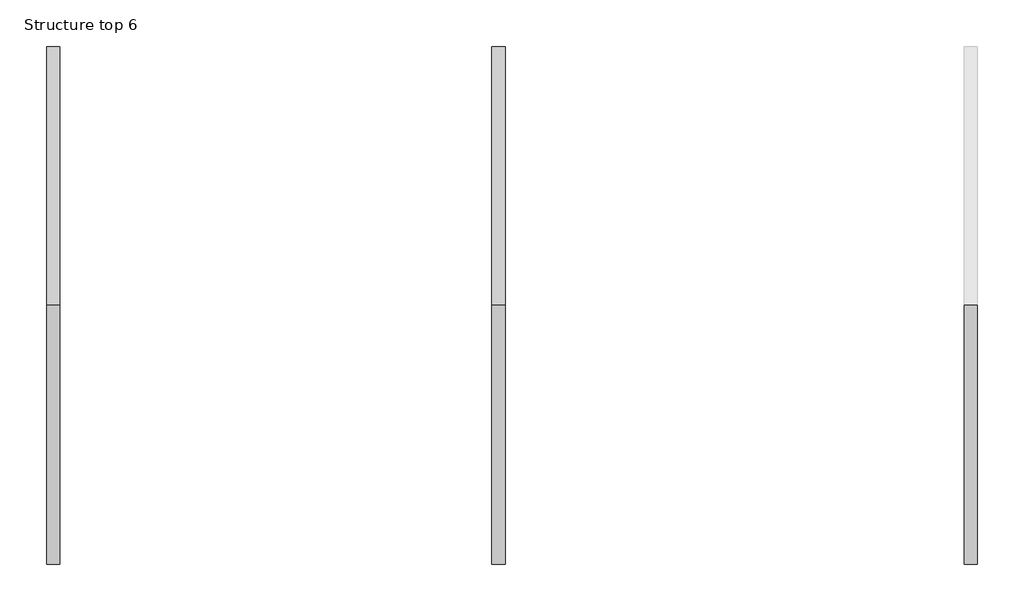
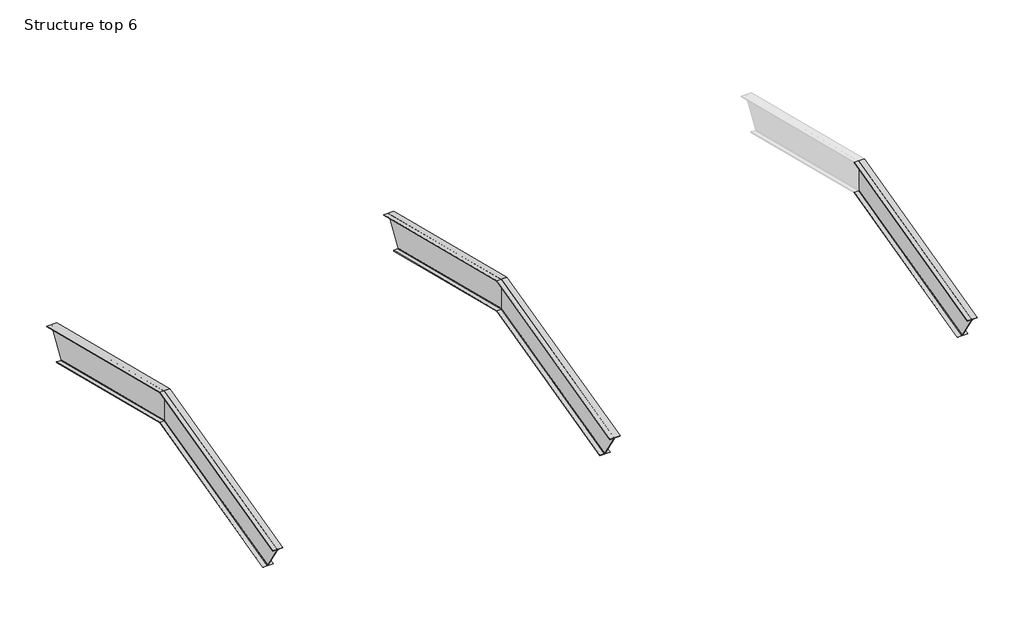
# One storey, part 1 of 2: 5 beams.
"""IFC4 building model written with IfcOpenShell, lengths in millimetres."""

import ifcopenshell
import ifcopenshell.guid

model = None  # the IFC model being written
_history = None  # IfcOwnerHistory: only IFC2X3 demands one
_inside = {}  # id of a spatial element -> (the spatial element, [elements in it])
_under = {}  # id of a project, library or spatial element -> (it, [spatial elements below it])
_declared = {}  # id of a project -> (the project, [libraries it declares])
_typed = {}  # id of a type object -> (the type object, [elements of that type])
_made_of = {}  # id of a material, layer set ... -> (it, [elements and type objects made of it])


def new_model(schema):
    """Start an empty IFC model of exactly this schema.

    Asked for "IFC4X3", IfcOpenShell would pick the latest addendum, in which some entities
    have other attributes; the version numbers below select the first issue.
    IFC2X3 requires an IfcOwnerHistory on every rooted entity: one is made here for all.
    """
    global model, _history
    if schema == "IFC4X3":
        model = ifcopenshell.file(schema_version=(4, 3, 0, 0))
    else:
        model = ifcopenshell.file(schema=schema)
    _inside.clear()
    _under.clear()
    _declared.clear()
    _typed.clear()
    _made_of.clear()
    _history = None
    if model.schema == "IFC2X3":
        org = make("IfcOrganization", Name="unknown")
        user = make(
            "IfcPersonAndOrganization",
            ThePerson=make("IfcPerson", FamilyName="unknown"),
            TheOrganization=org,
        )
        app = make(
            "IfcApplication",
            ApplicationDeveloper=org,
            Version="unknown",
            ApplicationFullName="unknown",
            ApplicationIdentifier="unknown",
        )
        _history = make(
            "IfcOwnerHistory",
            OwningUser=user,
            OwningApplication=app,
            ChangeAction="ADDED",
            CreationDate=0,
        )
    return model


def make(cls, **values):
    """One entity of the class cls with the attributes given. An attribute that is None is left unset."""
    return model.create_entity(
        cls, **{name: value for name, value in values.items() if value is not None}
    )


def rooted(cls, **values):
    """An entity with a GlobalId (a new one), such as an element, a storey or a relation."""
    return make(cls, GlobalId=ifcopenshell.guid.new(), OwnerHistory=_history, **values)


def si_unit(unit_type, name, prefix=None):
    """IfcSIUnit, for example si_unit("LENGTHUNIT", "METRE", prefix="MILLI")."""
    return make("IfcSIUnit", UnitType=unit_type, Prefix=prefix, Name=name)


def assignment(units):
    """IfcUnitAssignment: the units of a project."""
    return None if units is None else make("IfcUnitAssignment", Units=units)


def point(xyz):
    """IfcCartesianPoint."""
    return None if xyz is None else make("IfcCartesianPoint", Coordinates=xyz)


def direction(xyz):
    """IfcDirection."""
    return None if xyz is None else make("IfcDirection", DirectionRatios=xyz)


def frame(location, z_axis=None, x_axis=None):
    """IfcAxis2Placement3D, a coordinate frame: its origin and axes. An axis left out is left unset."""
    return make(
        "IfcAxis2Placement3D",
        Location=point(location),
        Axis=direction(z_axis),
        RefDirection=direction(x_axis),
    )


def origin():
    """The frame at (0, 0, 0) with its axes left unset."""
    return frame((0.0, 0.0, 0.0))


def place(relative_to, where):
    """IfcLocalPlacement: puts the frame where relative to a parent placement (None: the world)."""
    return make(
        "IfcLocalPlacement", PlacementRelTo=relative_to, RelativePlacement=where
    )


def context(
    kind, dimensions, precision=None, world=None, true_north=None, identifier=None
):
    """IfcGeometricRepresentationContext, for example the 3D "Model" context."""
    return make(
        "IfcGeometricRepresentationContext",
        ContextIdentifier=identifier,
        ContextType=kind,
        CoordinateSpaceDimension=dimensions,
        Precision=precision,
        WorldCoordinateSystem=world,
        TrueNorth=true_north,
    )


def project(units=None, contexts=None):
    """IfcProject with its units and contexts."""
    return rooted(
        "IfcProject",
        Name="project",
        RepresentationContexts=contexts,
        UnitsInContext=assignment(units),
    )


def spatial(cls, under=None, at=None, **own):
    """A site, building, storey or space (cls), placed at a placement, below another one or the project."""
    s = rooted(cls, ObjectPlacement=at, **own)
    if under is not None:
        _under.setdefault(under.id(), (under, []))[1].append(s)
    return s


def polyline(points):
    """IfcPolyline through the points."""
    return make("IfcPolyline", Points=[point(p) for p in points])


def ellipse_curve(where, semi_axis1, semi_axis2):
    """IfcEllipse in the frame where."""
    return make(
        "IfcEllipse", Position=where, SemiAxis1=semi_axis1, SemiAxis2=semi_axis2
    )


def shape(context_of_items, identifier, shape_type, items):
    """IfcShapeRepresentation: the items that make up one representation, for example the "Body"."""
    return make(
        "IfcShapeRepresentation",
        ContextOfItems=context_of_items,
        RepresentationIdentifier=identifier,
        RepresentationType=shape_type,
        Items=items,
    )


def made_of(thing, what):
    """Note that an element or type object is made of a material, layer set ...; save() writes the relation."""
    if what is not None:
        _made_of.setdefault(what.id(), (what, []))[1].append(thing)
    return thing


def element(
    cls,
    number,
    at=None,
    inside=None,
    cuts=None,
    type_object=None,
    material=None,
    context=None,
    identifier="Body",
    shape_type=None,
    held_by="IfcProductDefinitionShape",
    body=None,
    shapes=None,
    **own,
):
    """One element of the class cls, such as IfcWall. Its Tag is "e" and its number.

    at: its placement. inside: the storey or other place that contains it. cuts: it is an
    opening in that element (IfcRelVoidsElement). A single representation is given by context,
    identifier, shape_type and body (its items); several are given by shapes. held_by: the class
    of the entity that holds the representations. save() writes the other relations.
    """
    e = rooted(cls, Tag="e%d" % number, ObjectPlacement=at, **own)
    if body is not None:
        shapes = [shape(context, identifier, shape_type, body)]
    if shapes is not None:
        e.Representation = make(held_by, Representations=shapes)
    if inside is not None:
        _inside.setdefault(inside.id(), (inside, []))[1].append(e)
    if cuts is not None:
        rooted(
            "IfcRelVoidsElement", RelatingBuildingElement=cuts, RelatedOpeningElement=e
        )
    if type_object is not None:
        _typed.setdefault(type_object.id(), (type_object, []))[1].append(e)
    return made_of(e, material)


def aggregate(whole, parts):
    """IfcRelAggregates: a whole, such as a stair, and the parts it consists of."""
    return rooted("IfcRelAggregates", RelatingObject=whole, RelatedObjects=parts)


def save(model, path):
    """Write the relations noted so far, then the file.

    IfcRelAggregates (storeys below a building ...), IfcRelContainedInSpatialStructure (elements
    in a storey), IfcRelDefinesByType, IfcRelAssociatesMaterial and IfcRelDeclares: one each for
    every whole, place, type object, material and project.
    """
    for whole, parts in _under.values():
        aggregate(whole, parts)
    for where, things in _inside.values():
        rooted(
            "IfcRelContainedInSpatialStructure",
            RelatedElements=things,
            RelatingStructure=where,
        )
    for kind, things in _typed.values():
        rooted("IfcRelDefinesByType", RelatedObjects=things, RelatingType=kind)
    for what, things in _made_of.values():
        rooted("IfcRelAssociatesMaterial", RelatedObjects=things, RelatingMaterial=what)
    for by, libraries in _declared.values():
        rooted("IfcRelDeclares", RelatingContext=by, RelatedDefinitions=libraries)
    model.write(path)


def plane_surface(at):
    """IfcPlane: the flat surface through the origin of the frame at, square to its z axis."""
    return make("IfcPlane", Position=at)


def revolved_surface(curve, axis_point, axis_direction):
    """IfcSurfaceOfRevolution: the curve turned about the line through axis_point along axis_direction."""
    return make(
        "IfcSurfaceOfRevolution",
        SweptCurve=make("IfcArbitraryOpenProfileDef", ProfileType="CURVE", Curve=curve),
        AxisPosition=make("IfcAxis1Placement", Location=point(axis_point), Axis=direction(axis_direction)),
    )


def advanced_brep(points, edges, surfaces, faces):
    """IfcAdvancedBrep: a solid bounded by faces that lie on surfaces and meet in shared edges.

    An edge is (start, end): straight between two places in points (the first is 0);
    or (start, end, curve); or (start, end, curve, False) where it runs against its curve.
    A face is (place in surfaces, loops), or (place, loops, False) where it looks against
    its surface's normal. A loop lists edges by number (the first is 1), with a minus sign
    where the edge is run from its end to its start. The first loop is the outer one.
    """
    corners = [point(p) for p in points]
    vertices = [make("IfcVertexPoint", VertexGeometry=c) for c in corners]
    made = []
    for start, end, *more in edges:
        made.append(
            make(
                "IfcEdgeCurve",
                EdgeStart=vertices[start],
                EdgeEnd=vertices[end],
                EdgeGeometry=more[0] if more else make("IfcPolyline", Points=[corners[start], corners[end]]),
                SameSense=more[1] if len(more) > 1 else True,
            )
        )
    hull = []
    for where, loops, *sense in faces:
        bounds = []
        for j, loop in enumerate(loops):
            ring = [make("IfcOrientedEdge", EdgeElement=made[abs(k) - 1], Orientation=k > 0) for k in loop]
            bounds.append(
                make(
                    "IfcFaceOuterBound" if j == 0 else "IfcFaceBound",
                    Bound=make("IfcEdgeLoop", EdgeList=ring),
                    Orientation=True,
                )
            )
        hull.append(make("IfcAdvancedFace", Bounds=bounds, FaceSurface=surfaces[where], SameSense=sense[0] if sense else True))
    return make("IfcAdvancedBrep", Outer=make("IfcClosedShell", CfsFaces=hull))


model = new_model("IFC4")

# Units and contexts
model_context = context("Model", 3, world=origin())
ifc_project = project(units=[si_unit("LENGTHUNIT", "METRE", prefix="MILLI")], contexts=[model_context])

# Site, building, storey
site = spatial("IfcSite", under=ifc_project)
building = spatial("IfcBuilding", under=site)
storey = spatial("IfcBuildingStorey", under=building, Name="Structure top 6", Elevation=5867.6650904)

# Beams
placement = place(None, origin())
element("IfcBeam", 1, ObjectType="W Shapes : W 6X18.5", at=placement, inside=storey, context=model_context, shape_type="AdvancedBrep", body=[
    advanced_brep(
    [(12635.1244333, 7113.772024, 5183.7974927), (12700.7834333, 7113.772024, 5183.7974927), (12700.7834333, 9790.156119, 4514.7014689), (12635.1244333, 9790.156119, 4514.7014689), (12627.5044333, 7113.772024, 5191.6520089), (12627.5044333, 9794.417492, 4521.4906419), (12627.5044333, 7113.772024, 5640.4067021), (12627.5044333, 10037.8839324, 4909.378725), (12635.1244333, 7113.772024, 5648.2612183), (12635.1244333, 10042.1453053, 4916.1678979), (12700.7834333, 7113.772024, 5648.2612183), (12700.7834333, 10042.1453053, 4916.1678979), (12700.7834333, 7113.772024, 5658.2102722), (12700.7834333, 10047.5430444, 4924.7675171), (12548.3834333, 7113.772024, 5658.2102722), (12548.3834333, 10047.5430444, 4924.7675171), (12548.3834333, 7113.772024, 5648.2612183), (12548.3834333, 10042.1453053, 4916.1678979), (12614.0424333, 7113.772024, 5648.2612183), (12614.0424333, 10042.1453053, 4916.1678979), (12621.6624333, 7113.772024, 5640.4067021), (12621.6624333, 10037.8839324, 4909.378725), (12621.6624333, 7113.772024, 5191.6520089), (12621.6624333, 9794.417492, 4521.4906419), (12614.0424333, 7113.772024, 5183.7974927), (12614.0424333, 9790.156119, 4514.7014689), (12548.3834333, 7113.772024, 5183.7974927), (12548.3834333, 9790.156119, 4514.7014689), (12548.3834333, 7113.772024, 5173.8484388), (12548.3834333, 9784.75838, 4506.1018498), (12700.7834333, 7113.772024, 5173.8484388), (12700.7834333, 9784.75838, 4506.1018498)],
    [
        (0, 1),
        (1, 2),
        (2, 3),
        (3, 0),
        (4, 0, ellipse_curve(frame((12635.1244333, 7113.772024, 5191.6520089), z_axis=(0.0, -1.0, 0.0), x_axis=(0.0, 0.0, -1.0)), 7.8545162, 7.62)),
        (3, 5, ellipse_curve(frame((12635.1244333, 9794.417492, 4521.4906419), z_axis=(0.0, 0.8469796531886633, -0.5316253070390948), x_axis=(0.0, 0.531625307039094, 0.8469796531886635)), 8.0157451, 7.62)),
        (5, 4),
        (6, 4),
        (5, 7),
        (7, 6),
        (8, 6, ellipse_curve(frame((12635.1244333, 7113.772024, 5640.4067021), z_axis=(0.0, -1.0, 0.0), x_axis=(0.0, 0.0, -1.0)), 7.8545162, 7.62)),
        (7, 9, ellipse_curve(frame((12635.1244333, 10037.8839324, 4909.378725), z_axis=(0.0, 0.8469796531886633, -0.5316253070390948), x_axis=(0.0, 0.531625307039094, 0.8469796531886635)), 8.0157451, 7.62)),
        (9, 8),
        (10, 8),
        (9, 11),
        (11, 10),
        (12, 10),
        (11, 13),
        (13, 12),
        (14, 12),
        (13, 15),
        (15, 14),
        (16, 14),
        (15, 17),
        (17, 16),
        (18, 16),
        (17, 19),
        (19, 18),
        (20, 18, ellipse_curve(frame((12614.0424333, 7113.772024, 5640.4067021), z_axis=(0.0, -1.0, 0.0), x_axis=(0.0, 0.0, -1.0)), 7.8545162, 7.62)),
        (19, 21, ellipse_curve(frame((12614.0424333, 10037.8839324, 4909.378725), z_axis=(0.0, 0.8469796531886633, -0.5316253070390948), x_axis=(0.0, 0.531625307039094, 0.8469796531886635)), 8.0157451, 7.62)),
        (21, 20),
        (22, 20),
        (21, 23),
        (23, 22),
        (24, 22, ellipse_curve(frame((12614.0424333, 7113.772024, 5191.6520089), z_axis=(0.0, -1.0, 0.0), x_axis=(0.0, 0.0, -1.0)), 7.8545162, 7.62)),
        (23, 25, ellipse_curve(frame((12614.0424333, 9794.417492, 4521.4906419), z_axis=(0.0, 0.8469796531886633, -0.5316253070390948), x_axis=(0.0, 0.531625307039094, 0.8469796531886635)), 8.0157451, 7.62)),
        (25, 24),
        (26, 24),
        (25, 27),
        (27, 26),
        (28, 26),
        (27, 29),
        (29, 28),
        (30, 28),
        (29, 31),
        (31, 30),
        (1, 30),
        (31, 2),
    ],
    [
        plane_surface(frame((12700.7834333, 7002.1447176, 5211.7043193), z_axis=(0.0, 0.24253562503633289, 0.9701425001453319), x_axis=(0.0, 0.9701425001453319, -0.24253562503633289))),
        revolved_surface(polyline([(12627.504433299999, 9796.830743469387, 4520.887328982653), (12627.504433299999, 7111.923902529412, 5192.114039217647)]), (12635.1244333, 7003.992839, 5219.0968051), (0.0, 0.9701425001453319, -0.24253562503633289)),
        plane_surface(frame((12627.5044333, 7003.992839, 5219.0968051), z_axis=(1.0, 0.0, 0.0), x_axis=(0.0, 0.9701425001453319, -0.24253562503633289))),
        revolved_surface(polyline([(12627.504433299999, 10040.297183869387, 4908.775412082653), (12627.504433299999, 7111.923902529412, 5640.868732417647)]), (12635.1244333, 7109.5821786, 5641.4541634), (0.0, 0.9701425001453319, -0.24253562503633289)),
        plane_surface(frame((12635.1244333, 7111.4303001, 5648.8466493), z_axis=(0.0, -0.24253562503633289, -0.9701425001453319), x_axis=(0.0, 0.9701425001453319, -0.24253562503633289))),
        plane_surface(frame((12700.7834333, 7111.4303001, 5648.8466493), z_axis=(1.0, 0.0, 0.0), x_axis=(0.0, 0.9701425001453319, -0.24253562503633289))),
        plane_surface(frame((12700.7834333, 7113.7712539, 5658.2104647), z_axis=(0.0, 0.24253562503633289, 0.9701425001453319), x_axis=(0.0, 0.9701425001453319, -0.24253562503633289))),
        plane_surface(frame((12548.3834333, 7113.7712539, 5658.2104647), z_axis=(-1.0, 0.0, 0.0), x_axis=(0.0, 0.9701425001453319, -0.24253562503633289))),
        plane_surface(frame((12548.3834333, 7111.4303001, 5648.8466493), z_axis=(0.0, -0.24253562503633289, -0.9701425001453319), x_axis=(0.0, 0.9701425001453319, -0.24253562503633289))),
        revolved_surface(polyline([(12606.422433299998, 10040.297183869387, 4908.775412082653), (12606.422433299998, 7111.923902529412, 5640.868732417647)]), (12614.0424333, 7109.5821786, 5641.4541634), (0.0, 0.9701425001453319, -0.24253562503633289)),
        plane_surface(frame((12621.6624333, 7109.5821786, 5641.4541634), z_axis=(-1.0, 0.0, 0.0), x_axis=(0.0, 0.9701425001453319, -0.24253562503633289))),
        revolved_surface(polyline([(12606.422433299998, 9796.830743469387, 4520.887328982653), (12606.422433299998, 7111.923902529412, 5192.114039217647)]), (12614.0424333, 7003.992839, 5219.0968051), (0.0, 0.9701425001453319, -0.24253562503633289)),
        plane_surface(frame((12614.0424333, 7002.1447176, 5211.7043193), z_axis=(0.0, 0.24253562503633289, 0.9701425001453319), x_axis=(0.0, 0.9701425001453319, -0.24253562503633289))),
        plane_surface(frame((12548.3834333, 7002.1447176, 5211.7043193), z_axis=(-1.0, 0.0, 0.0), x_axis=(0.0, 0.9701425001453319, -0.24253562503633289))),
        plane_surface(frame((12548.3834333, 6999.8037637, 5202.3405039), z_axis=(0.0, -0.24253562503633289, -0.9701425001453319), x_axis=(0.0, 0.9701425001453319, -0.24253562503633289))),
        plane_surface(frame((12700.7834333, 6999.8037637, 5202.3405039), z_axis=(1.0, 0.0, 0.0), x_axis=(0.0, 0.9701425001453319, -0.24253562503633289))),
        plane_surface(frame((12624.5870052, 7113.772024, 5658.2135449), z_axis=(0.0, -1.0, 0.0), x_axis=(0.0, 0.0, 1.0))),
        plane_surface(frame((12624.5870052, 10047.54482, 4924.7703459), z_axis=(0.0, 0.8469796531886633, -0.5316253070390948), x_axis=(1.0, 0.0, 0.0))),
    ],
    [
        (0, [[1, 2, 3, 4]]),
        (1, [[5, -4, 6, 7]]),
        (2, [[8, -7, 9, 10]]),
        (3, [[11, -10, 12, 13]]),
        (4, [[14, -13, 15, 16]]),
        (5, [[17, -16, 18, 19]]),
        (6, [[20, -19, 21, 22]]),
        (7, [[23, -22, 24, 25]]),
        (8, [[26, -25, 27, 28]]),
        (9, [[29, -28, 30, 31]]),
        (10, [[32, -31, 33, 34]]),
        (11, [[35, -34, 36, 37]]),
        (12, [[38, -37, 39, 40]]),
        (13, [[41, -40, 42, 43]]),
        (14, [[44, -43, 45, 46]]),
        (15, [[47, -46, 48, -2]]),
        (16, [[-1, -5, -8, -11, -14, -17, -20, -23, -26, -29, -32, -35, -38, -41, -44, -47]]),
        (17, [[-48, -45, -42, -39, -36, -33, -30, -27, -24, -21, -18, -15, -12, -9, -6, -3]]),
    ],
),
])
element("IfcBeam", 2, ObjectType="W Shapes : W 6X18.5", at=placement, inside=storey, context=model_context, shape_type="AdvancedBrep", body=[
    advanced_brep(
    [(12635.1244333, 4437.3879289, 4514.7014689), (12700.7834333, 4437.3879289, 4514.7014689), (12700.7834333, 7113.772024, 5183.7974927), (12635.1244333, 7113.772024, 5183.7974927), (12627.5044333, 4433.1265559, 4521.4906419), (12627.5044333, 7113.772024, 5191.6520089), (12627.5044333, 4189.6601155, 4909.378725), (12627.5044333, 7113.772024, 5640.4067021), (12635.1244333, 4185.3987426, 4916.1678979), (12635.1244333, 7113.772024, 5648.2612183), (12700.7834333, 4185.3987426, 4916.1678979), (12700.7834333, 7113.772024, 5648.2612183), (12700.7834333, 4180.0010035, 4924.7675171), (12700.7834333, 7113.772024, 5658.2102722), (12548.3834333, 4180.0010035, 4924.7675171), (12548.3834333, 7113.772024, 5658.2102722), (12548.3834333, 4185.3987426, 4916.1678979), (12548.3834333, 7113.772024, 5648.2612183), (12614.0424333, 4185.3987426, 4916.1678979), (12614.0424333, 7113.772024, 5648.2612183), (12621.6624333, 4189.6601155, 4909.378725), (12621.6624333, 7113.772024, 5640.4067021), (12621.6624333, 4433.1265559, 4521.4906419), (12621.6624333, 7113.772024, 5191.6520089), (12614.0424333, 4437.3879289, 4514.7014689), (12614.0424333, 7113.772024, 5183.7974927), (12548.3834333, 4437.3879289, 4514.7014689), (12548.3834333, 7113.772024, 5183.7974927), (12548.3834333, 4442.7856679, 4506.1018498), (12548.3834333, 7113.772024, 5173.8484388), (12700.7834333, 4442.7856679, 4506.1018498), (12700.7834333, 7113.772024, 5173.8484388)],
    [
        (0, 1),
        (1, 2),
        (2, 3),
        (3, 0),
        (4, 0, ellipse_curve(frame((12635.1244333, 4433.1265559, 4521.4906419), z_axis=(0.0, -0.8469796531886659, -0.5316253070390907), x_axis=(0.0, 0.5316253070390901, -0.8469796531886661)), 8.0157451, 7.62)),
        (3, 5, ellipse_curve(frame((12635.1244333, 7113.772024, 5191.6520089), z_axis=(0.0, 1.0, 0.0), x_axis=(0.0, 0.0, 0.9999999999999999)), 7.8545162, 7.62)),
        (5, 4),
        (6, 4),
        (5, 7),
        (7, 6),
        (8, 6, ellipse_curve(frame((12635.1244333, 4189.6601155, 4909.378725), z_axis=(0.0, -0.8469796531886659, -0.5316253070390907), x_axis=(0.0, 0.5316253070390901, -0.8469796531886661)), 8.0157451, 7.62)),
        (7, 9, ellipse_curve(frame((12635.1244333, 7113.772024, 5640.4067021), z_axis=(0.0, 1.0, 0.0), x_axis=(0.0, 0.0, 0.9999999999999999)), 7.8545162, 7.62)),
        (9, 8),
        (10, 8),
        (9, 11),
        (11, 10),
        (12, 10),
        (11, 13),
        (13, 12),
        (14, 12),
        (13, 15),
        (15, 14),
        (16, 14),
        (15, 17),
        (17, 16),
        (18, 16),
        (17, 19),
        (19, 18),
        (20, 18, ellipse_curve(frame((12614.0424333, 4189.6601155, 4909.378725), z_axis=(0.0, -0.8469796531886659, -0.5316253070390907), x_axis=(0.0, 0.5316253070390901, -0.8469796531886661)), 8.0157451, 7.62)),
        (19, 21, ellipse_curve(frame((12614.0424333, 7113.772024, 5640.4067021), z_axis=(0.0, 1.0, 0.0), x_axis=(0.0, 0.0, 0.9999999999999999)), 7.8545162, 7.62)),
        (21, 20),
        (22, 20),
        (21, 23),
        (23, 22),
        (24, 22, ellipse_curve(frame((12614.0424333, 4433.1265559, 4521.4906419), z_axis=(0.0, -0.8469796531886659, -0.5316253070390907), x_axis=(0.0, 0.5316253070390901, -0.8469796531886661)), 8.0157451, 7.62)),
        (23, 25, ellipse_curve(frame((12614.0424333, 7113.772024, 5191.6520089), z_axis=(0.0, 1.0, 0.0), x_axis=(0.0, 0.0, 0.9999999999999999)), 7.8545162, 7.62)),
        (25, 24),
        (26, 24),
        (25, 27),
        (27, 26),
        (28, 26),
        (27, 29),
        (29, 28),
        (30, 28),
        (29, 31),
        (31, 30),
        (1, 30),
        (31, 2),
    ],
    [
        plane_surface(frame((12700.7834333, 4291.6265344, 4478.2611203), z_axis=(0.0, -0.2425356250363261, 0.9701425001453337), x_axis=(0.0, 0.9701425001453337, 0.2425356250363261))),
        revolved_surface(polyline([(12627.504433299999, 7115.620145464711, 5192.114039241156), (12627.504433299999, 4430.713304430615, 4520.887328982652)]), (12635.1244333, 4289.7784129, 4485.6536061), (0.0, 0.9701425001453337, 0.2425356250363261)),
        plane_surface(frame((12627.5044333, 4289.7784129, 4485.6536061), z_axis=(1.0, 0.0, 0.0), x_axis=(0.0, 0.9701425001453337, 0.2425356250363261))),
        revolved_surface(polyline([(12627.504433299999, 7115.620145464711, 5640.868732441156), (12627.504433299999, 4187.246864030613, 4908.775412082654)]), (12635.1244333, 4184.1890733, 4908.0109644), (0.0, 0.9701425001453337, 0.2425356250363261)),
        plane_surface(frame((12635.1244333, 4182.3409519, 4915.4034503), z_axis=(0.0, 0.2425356250363261, -0.9701425001453337), x_axis=(0.0, 0.9701425001453337, 0.2425356250363261))),
        plane_surface(frame((12700.7834333, 4182.3409519, 4915.4034503), z_axis=(1.0, 0.0, 0.0), x_axis=(0.0, 0.9701425001453337, 0.2425356250363261))),
        plane_surface(frame((12700.7834333, 4179.999998, 4924.7672657), z_axis=(0.0, -0.2425356250363261, 0.9701425001453337), x_axis=(0.0, 0.9701425001453337, 0.2425356250363261))),
        plane_surface(frame((12548.3834333, 4179.999998, 4924.7672657), z_axis=(-1.0, 0.0, 0.0), x_axis=(0.0, 0.9701425001453337, 0.2425356250363261))),
        plane_surface(frame((12548.3834333, 4182.3409519, 4915.4034503), z_axis=(0.0, 0.2425356250363261, -0.9701425001453337), x_axis=(0.0, 0.9701425001453337, 0.2425356250363261))),
        revolved_surface(polyline([(12606.422433299998, 7115.620145464711, 5640.868732441156), (12606.422433299998, 4187.246864030613, 4908.775412082654)]), (12614.0424333, 4184.1890733, 4908.0109644), (0.0, 0.9701425001453337, 0.2425356250363261)),
        plane_surface(frame((12621.6624333, 4184.1890733, 4908.0109644), z_axis=(-1.0, 0.0, 0.0), x_axis=(0.0, 0.9701425001453337, 0.2425356250363261))),
        revolved_surface(polyline([(12606.422433299998, 7115.620145464711, 5192.114039241156), (12606.422433299998, 4430.713304430615, 4520.887328982652)]), (12614.0424333, 4289.7784129, 4485.6536061), (0.0, 0.9701425001453337, 0.2425356250363261)),
        plane_surface(frame((12614.0424333, 4291.6265344, 4478.2611203), z_axis=(0.0, -0.2425356250363261, 0.9701425001453337), x_axis=(0.0, 0.9701425001453337, 0.2425356250363261))),
        plane_surface(frame((12548.3834333, 4291.6265344, 4478.2611203), z_axis=(-1.0, 0.0, 0.0), x_axis=(0.0, 0.9701425001453337, 0.2425356250363261))),
        plane_surface(frame((12548.3834333, 4293.9674882, 4468.8973049), z_axis=(0.0, 0.2425356250363261, -0.9701425001453337), x_axis=(0.0, 0.9701425001453337, 0.2425356250363261))),
        plane_surface(frame((12700.7834333, 4293.9674882, 4468.8973049), z_axis=(1.0, 0.0, 0.0), x_axis=(0.0, 0.9701425001453337, 0.2425356250363261))),
        plane_surface(frame((12624.5870052, 7113.772024, 5658.2135449), z_axis=(0.0, 1.0, 0.0), x_axis=(0.0, 0.0, -1.0))),
        plane_surface(frame((12624.5870052, 4179.999228, 4924.7703459), z_axis=(0.0, -0.8469796531886659, -0.5316253070390907), x_axis=(1.0, 0.0, 0.0))),
    ],
    [
        (0, [[1, 2, 3, 4]]),
        (1, [[5, -4, 6, 7]]),
        (2, [[8, -7, 9, 10]]),
        (3, [[11, -10, 12, 13]]),
        (4, [[14, -13, 15, 16]]),
        (5, [[17, -16, 18, 19]]),
        (6, [[20, -19, 21, 22]]),
        (7, [[23, -22, 24, 25]]),
        (8, [[26, -25, 27, 28]]),
        (9, [[29, -28, 30, 31]]),
        (10, [[32, -31, 33, 34]]),
        (11, [[35, -34, 36, 37]]),
        (12, [[38, -37, 39, 40]]),
        (13, [[41, -40, 42, 43]]),
        (14, [[44, -43, 45, 46]]),
        (15, [[47, -46, 48, -2]]),
        (16, [[-48, -45, -42, -39, -36, -33, -30, -27, -24, -21, -18, -15, -12, -9, -6, -3]]),
        (17, [[-1, -5, -8, -11, -14, -17, -20, -23, -26, -29, -32, -35, -38, -41, -44, -47]]),
    ],
),
])
element("IfcBeam", 3, ObjectType="W Shapes : W 6X18.5", at=placement, inside=storey, context=model_context, shape_type="AdvancedBrep", body=[
    advanced_brep(
    [(7586.8744333, 7113.772024, 5183.7974927), (7652.5334333, 7113.772024, 5183.7974927), (7652.5334333, 9790.156119, 4514.7014689), (7586.8744333, 9790.156119, 4514.7014689), (7579.2544333, 7113.772024, 5191.6520089), (7579.2544333, 9794.417492, 4521.4906419), (7579.2544333, 7113.772024, 5640.4067021), (7579.2544333, 10037.8839324, 4909.378725), (7586.8744333, 7113.772024, 5648.2612183), (7586.8744333, 10042.1453053, 4916.1678979), (7652.5334333, 7113.772024, 5648.2612183), (7652.5334333, 10042.1453053, 4916.1678979), (7652.5334333, 7113.772024, 5658.2102722), (7652.5334333, 10047.5430444, 4924.7675171), (7500.1334333, 7113.772024, 5658.2102722), (7500.1334333, 10047.5430444, 4924.7675171), (7500.1334333, 7113.772024, 5648.2612183), (7500.1334333, 10042.1453053, 4916.1678979), (7565.7924333, 7113.772024, 5648.2612183), (7565.7924333, 10042.1453053, 4916.1678979), (7573.4124333, 7113.772024, 5640.4067021), (7573.4124333, 10037.8839324, 4909.378725), (7573.4124333, 7113.772024, 5191.6520089), (7573.4124333, 9794.417492, 4521.4906419), (7565.7924333, 7113.772024, 5183.7974927), (7565.7924333, 9790.156119, 4514.7014689), (7500.1334333, 7113.772024, 5183.7974927), (7500.1334333, 9790.156119, 4514.7014689), (7500.1334333, 7113.772024, 5173.8484388), (7500.1334333, 9784.75838, 4506.1018498), (7652.5334333, 7113.772024, 5173.8484388), (7652.5334333, 9784.75838, 4506.1018498)],
    [
        (0, 1),
        (1, 2),
        (2, 3),
        (3, 0),
        (4, 0, ellipse_curve(frame((7586.8744333, 7113.772024, 5191.6520089), z_axis=(0.0, -1.0, 0.0), x_axis=(0.0, 0.0, -1.0)), 7.8545162, 7.62)),
        (3, 5, ellipse_curve(frame((7586.8744333, 9794.417492, 4521.4906419), z_axis=(0.0, 0.8469796531886629, -0.5316253070390953), x_axis=(0.0, 0.5316253070390956, 0.8469796531886628)), 8.0157451, 7.62)),
        (5, 4),
        (6, 4),
        (5, 7),
        (7, 6),
        (8, 6, ellipse_curve(frame((7586.8744333, 7113.772024, 5640.4067021), z_axis=(0.0, -1.0, 0.0), x_axis=(0.0, 0.0, -1.0)), 7.8545162, 7.62)),
        (7, 9, ellipse_curve(frame((7586.8744333, 10037.8839324, 4909.378725), z_axis=(0.0, 0.8469796531886629, -0.5316253070390953), x_axis=(0.0, 0.5316253070390956, 0.8469796531886628)), 8.0157451, 7.62)),
        (9, 8),
        (10, 8),
        (9, 11),
        (11, 10),
        (12, 10),
        (11, 13),
        (13, 12),
        (14, 12),
        (13, 15),
        (15, 14),
        (16, 14),
        (15, 17),
        (17, 16),
        (18, 16),
        (17, 19),
        (19, 18),
        (20, 18, ellipse_curve(frame((7565.7924333, 7113.772024, 5640.4067021), z_axis=(0.0, -1.0, 0.0), x_axis=(0.0, 0.0, -1.0)), 7.8545162, 7.62)),
        (19, 21, ellipse_curve(frame((7565.7924333, 10037.8839324, 4909.378725), z_axis=(0.0, 0.8469796531886629, -0.5316253070390953), x_axis=(0.0, 0.5316253070390956, 0.8469796531886628)), 8.0157451, 7.62)),
        (21, 20),
        (22, 20),
        (21, 23),
        (23, 22),
        (24, 22, ellipse_curve(frame((7565.7924333, 7113.772024, 5191.6520089), z_axis=(0.0, -1.0, 0.0), x_axis=(0.0, 0.0, -1.0)), 7.8545162, 7.62)),
        (23, 25, ellipse_curve(frame((7565.7924333, 9794.417492, 4521.4906419), z_axis=(0.0, 0.8469796531886629, -0.5316253070390953), x_axis=(0.0, 0.5316253070390956, 0.8469796531886628)), 8.0157451, 7.62)),
        (25, 24),
        (26, 24),
        (25, 27),
        (27, 26),
        (28, 26),
        (27, 29),
        (29, 28),
        (30, 28),
        (29, 31),
        (31, 30),
        (1, 30),
        (31, 2),
    ],
    [
        plane_surface(frame((7619.7039333, 7002.1447176, 5211.7043193), z_axis=(0.0, 0.24253562503633289, 0.9701425001453319), x_axis=(-1.0, 0.0, 0.0))),
        revolved_surface(polyline([(7579.2544333000005, 9796.830743469387, 4520.887328982653), (7579.2544333000005, 7111.923902529412, 5192.114039217647)]), (7586.8744333, 7003.992839, 5219.0968051), (0.0, 0.9701425001453319, -0.24253562503633289)),
        plane_surface(frame((7579.2544333, 7056.7875088, 5430.2754843), z_axis=(1.0, 0.0, 0.0), x_axis=(0.0, 0.24253562503633308, 0.9701425001453319))),
        revolved_surface(polyline([(7586.8744333, 10042.145305332164, 4916.16789793376), (7586.8744333, 7113.772023992189, 5648.261218268754)]), (7586.8744333, 7109.5821786, 5641.4541634), (0.0, 0.9701425001453319, -0.24253562503633289)),
        plane_surface(frame((7619.7039333, 7111.4303001, 5648.8466493), z_axis=(0.0, -0.24253562503633289, -0.9701425001453319), x_axis=(1.0, 0.0, 0.0))),
        plane_surface(frame((7652.5334333, 7112.600777, 5653.528557), z_axis=(1.0, 0.0, 0.0), x_axis=(0.0, 0.24253562503633308, 0.9701425001453319))),
        plane_surface(frame((7576.3334333, 7113.7712539, 5658.2104647), z_axis=(0.0, 0.24253562503633289, 0.9701425001453319), x_axis=(-1.0, 0.0, 0.0))),
        plane_surface(frame((7500.1334333, 7112.600777, 5653.528557), z_axis=(-1.0, 0.0, 0.0), x_axis=(0.0, -0.24253562503633308, -0.9701425001453319))),
        plane_surface(frame((7532.9629333, 7111.4303001, 5648.8466493), z_axis=(0.0, -0.24253562503633289, -0.9701425001453319), x_axis=(1.0, 0.0, 0.0))),
        revolved_surface(polyline([(7573.4124333, 10040.297183869387, 4908.775412082653), (7573.4124333, 7111.923902529412, 5640.868732417647)]), (7565.7924333, 7109.5821786, 5641.4541634), (0.0, 0.9701425001453319, -0.24253562503633289)),
        plane_surface(frame((7573.4124333, 7056.7875088, 5430.2754843), z_axis=(-1.0, 0.0, 0.0), x_axis=(0.0, -0.24253562503633308, -0.9701425001453319))),
        revolved_surface(polyline([(7565.7924333, 9794.98262200661, 4513.494843131546), (7565.7924333, 7110.075781066635, 5184.721553366539)]), (7565.7924333, 7003.992839, 5219.0968051), (0.0, 0.9701425001453319, -0.24253562503633289)),
        plane_surface(frame((7532.9629333, 7002.1447176, 5211.7043193), z_axis=(0.0, 0.24253562503633289, 0.9701425001453319), x_axis=(-1.0, 0.0, 0.0))),
        plane_surface(frame((7500.1334333, 7000.9742406, 5207.0224116), z_axis=(-1.0, 0.0, 0.0), x_axis=(0.0, -0.24253562503633308, -0.9701425001453319))),
        plane_surface(frame((7576.3334333, 6999.8037637, 5202.3405039), z_axis=(0.0, -0.24253562503633289, -0.9701425001453319), x_axis=(1.0, 0.0, 0.0))),
        plane_surface(frame((7652.5334333, 7000.9742406, 5207.0224116), z_axis=(1.0, 0.0, 0.0), x_axis=(0.0, 0.24253562503633308, 0.9701425001453319))),
        plane_surface(frame((7576.3370052, 7113.772024, 5658.2135449), z_axis=(0.0, -1.0, 0.0), x_axis=(0.0, 0.0, 1.0))),
        plane_surface(frame((7576.3370052, 10047.54482, 4924.7703459), z_axis=(0.0, 0.8469796531886629, -0.5316253070390953), x_axis=(1.0, 0.0, 0.0))),
    ],
    [
        (0, [[1, 2, 3, 4]]),
        (1, [[5, -4, 6, 7]]),
        (2, [[8, -7, 9, 10]]),
        (3, [[11, -10, 12, 13]]),
        (4, [[14, -13, 15, 16]]),
        (5, [[17, -16, 18, 19]]),
        (6, [[20, -19, 21, 22]]),
        (7, [[23, -22, 24, 25]]),
        (8, [[26, -25, 27, 28]]),
        (9, [[29, -28, 30, 31]]),
        (10, [[32, -31, 33, 34]]),
        (11, [[35, -34, 36, 37]]),
        (12, [[38, -37, 39, 40]]),
        (13, [[41, -40, 42, 43]]),
        (14, [[44, -43, 45, 46]]),
        (15, [[47, -46, 48, -2]]),
        (16, [[-1, -5, -8, -11, -14, -17, -20, -23, -26, -29, -32, -35, -38, -41, -44, -47]]),
        (17, [[-48, -45, -42, -39, -36, -33, -30, -27, -24, -21, -18, -15, -12, -9, -6, -3]]),
    ],
),
])
element("IfcBeam", 4, ObjectType="W Shapes : W 6X18.5", at=placement, inside=storey, context=model_context, shape_type="AdvancedBrep", body=[
    advanced_brep(
    [(7586.8744333, 4437.3879289, 4514.7014689), (7652.5334333, 4437.3879289, 4514.7014689), (7652.5334333, 7113.772024, 5183.7974927), (7586.8744333, 7113.772024, 5183.7974927), (7579.2544333, 4433.1265559, 4521.4906419), (7579.2544333, 7113.772024, 5191.6520089), (7579.2544333, 4189.6601155, 4909.378725), (7579.2544333, 7113.772024, 5640.4067021), (7586.8744333, 4185.3987426, 4916.1678979), (7586.8744333, 7113.772024, 5648.2612183), (7652.5334333, 4185.3987426, 4916.1678979), (7652.5334333, 7113.772024, 5648.2612183), (7652.5334333, 4180.0010035, 4924.7675171), (7652.5334333, 7113.772024, 5658.2102722), (7500.1334333, 4180.0010035, 4924.7675171), (7500.1334333, 7113.772024, 5658.2102722), (7500.1334333, 4185.3987426, 4916.1678979), (7500.1334333, 7113.772024, 5648.2612183), (7565.7924333, 4185.3987426, 4916.1678979), (7565.7924333, 7113.772024, 5648.2612183), (7573.4124333, 4189.6601155, 4909.378725), (7573.4124333, 7113.772024, 5640.4067021), (7573.4124333, 4433.1265559, 4521.4906419), (7573.4124333, 7113.772024, 5191.6520089), (7565.7924333, 4437.3879289, 4514.7014689), (7565.7924333, 7113.772024, 5183.7974927), (7500.1334333, 4437.3879289, 4514.7014689), (7500.1334333, 7113.772024, 5183.7974927), (7500.1334333, 4442.7856679, 4506.1018498), (7500.1334333, 7113.772024, 5173.8484388), (7652.5334333, 4442.7856679, 4506.1018498), (7652.5334333, 7113.772024, 5173.8484388)],
    [
        (0, 1),
        (1, 2),
        (2, 3),
        (3, 0),
        (4, 0, ellipse_curve(frame((7586.8744333, 4433.1265559, 4521.4906419), z_axis=(0.0, -0.8469796531886659, -0.5316253070390907), x_axis=(0.0, 0.5316253070390901, -0.8469796531886661)), 8.0157451, 7.62)),
        (3, 5, ellipse_curve(frame((7586.8744333, 7113.772024, 5191.6520089), z_axis=(0.0, 1.0, 0.0), x_axis=(0.0, 0.0, 0.9999999999999999)), 7.8545162, 7.62)),
        (5, 4),
        (6, 4),
        (5, 7),
        (7, 6),
        (8, 6, ellipse_curve(frame((7586.8744333, 4189.6601155, 4909.378725), z_axis=(0.0, -0.8469796531886659, -0.5316253070390907), x_axis=(0.0, 0.5316253070390901, -0.8469796531886661)), 8.0157451, 7.62)),
        (7, 9, ellipse_curve(frame((7586.8744333, 7113.772024, 5640.4067021), z_axis=(0.0, 1.0, 0.0), x_axis=(0.0, 0.0, 0.9999999999999999)), 7.8545162, 7.62)),
        (9, 8),
        (10, 8),
        (9, 11),
        (11, 10),
        (12, 10),
        (11, 13),
        (13, 12),
        (14, 12),
        (13, 15),
        (15, 14),
        (16, 14),
        (15, 17),
        (17, 16),
        (18, 16),
        (17, 19),
        (19, 18),
        (20, 18, ellipse_curve(frame((7565.7924333, 4189.6601155, 4909.378725), z_axis=(0.0, -0.8469796531886659, -0.5316253070390907), x_axis=(0.0, 0.5316253070390901, -0.8469796531886661)), 8.0157451, 7.62)),
        (19, 21, ellipse_curve(frame((7565.7924333, 7113.772024, 5640.4067021), z_axis=(0.0, 1.0, 0.0), x_axis=(0.0, 0.0, 0.9999999999999999)), 7.8545162, 7.62)),
        (21, 20),
        (22, 20),
        (21, 23),
        (23, 22),
        (24, 22, ellipse_curve(frame((7565.7924333, 4433.1265559, 4521.4906419), z_axis=(0.0, -0.8469796531886659, -0.5316253070390907), x_axis=(0.0, 0.5316253070390901, -0.8469796531886661)), 8.0157451, 7.62)),
        (23, 25, ellipse_curve(frame((7565.7924333, 7113.772024, 5191.6520089), z_axis=(0.0, 1.0, 0.0), x_axis=(0.0, 0.0, 0.9999999999999999)), 7.8545162, 7.62)),
        (25, 24),
        (26, 24),
        (25, 27),
        (27, 26),
        (28, 26),
        (27, 29),
        (29, 28),
        (30, 28),
        (29, 31),
        (31, 30),
        (1, 30),
        (31, 2),
    ],
    [
        plane_surface(frame((7652.5334333, 4291.6265344, 4478.2611203), z_axis=(0.0, -0.2425356250363261, 0.9701425001453337), x_axis=(0.0, 0.9701425001453337, 0.2425356250363261))),
        revolved_surface(polyline([(7579.2544333000005, 7115.620145464711, 5192.114039241156), (7579.2544333000005, 4430.713304430615, 4520.887328982652)]), (7586.8744333, 4289.7784129, 4485.6536061), (0.0, 0.9701425001453337, 0.2425356250363261)),
        plane_surface(frame((7579.2544333, 4289.7784129, 4485.6536061), z_axis=(1.0, 0.0, 0.0), x_axis=(0.0, 0.9701425001453337, 0.2425356250363261))),
        revolved_surface(polyline([(7579.2544333000005, 7115.620145464711, 5640.868732441156), (7579.2544333000005, 4187.246864030613, 4908.775412082654)]), (7586.8744333, 4184.1890733, 4908.0109644), (0.0, 0.9701425001453337, 0.2425356250363261)),
        plane_surface(frame((7586.8744333, 4182.3409519, 4915.4034503), z_axis=(0.0, 0.2425356250363261, -0.9701425001453337), x_axis=(0.0, 0.9701425001453337, 0.2425356250363261))),
        plane_surface(frame((7652.5334333, 4182.3409519, 4915.4034503), z_axis=(1.0, 0.0, 0.0), x_axis=(0.0, 0.9701425001453337, 0.2425356250363261))),
        plane_surface(frame((7652.5334333, 4179.999998, 4924.7672657), z_axis=(0.0, -0.2425356250363261, 0.9701425001453337), x_axis=(0.0, 0.9701425001453337, 0.2425356250363261))),
        plane_surface(frame((7500.1334333, 4179.999998, 4924.7672657), z_axis=(-1.0, 0.0, 0.0), x_axis=(0.0, 0.9701425001453337, 0.2425356250363261))),
        plane_surface(frame((7500.1334333, 4182.3409519, 4915.4034503), z_axis=(0.0, 0.2425356250363261, -0.9701425001453337), x_axis=(0.0, 0.9701425001453337, 0.2425356250363261))),
        revolved_surface(polyline([(7558.1724333, 7115.620145464711, 5640.868732441156), (7558.1724333, 4187.246864030613, 4908.775412082654)]), (7565.7924333, 4184.1890733, 4908.0109644), (0.0, 0.9701425001453337, 0.2425356250363261)),
        plane_surface(frame((7573.4124333, 4184.1890733, 4908.0109644), z_axis=(-1.0, 0.0, 0.0), x_axis=(0.0, 0.9701425001453337, 0.2425356250363261))),
        revolved_surface(polyline([(7558.1724333, 7115.620145464711, 5192.114039241156), (7558.1724333, 4430.713304430615, 4520.887328982652)]), (7565.7924333, 4289.7784129, 4485.6536061), (0.0, 0.9701425001453337, 0.2425356250363261)),
        plane_surface(frame((7565.7924333, 4291.6265344, 4478.2611203), z_axis=(0.0, -0.2425356250363261, 0.9701425001453337), x_axis=(0.0, 0.9701425001453337, 0.2425356250363261))),
        plane_surface(frame((7500.1334333, 4291.6265344, 4478.2611203), z_axis=(-1.0, 0.0, 0.0), x_axis=(0.0, 0.9701425001453337, 0.2425356250363261))),
        plane_surface(frame((7500.1334333, 4293.9674882, 4468.8973049), z_axis=(0.0, 0.2425356250363261, -0.9701425001453337), x_axis=(0.0, 0.9701425001453337, 0.2425356250363261))),
        plane_surface(frame((7652.5334333, 4293.9674882, 4468.8973049), z_axis=(1.0, 0.0, 0.0), x_axis=(0.0, 0.9701425001453337, 0.2425356250363261))),
        plane_surface(frame((7576.3370052, 7113.772024, 5658.2135449), z_axis=(0.0, 1.0, 0.0), x_axis=(0.0, 0.0, -1.0))),
        plane_surface(frame((7576.3370052, 4179.999228, 4924.7703459), z_axis=(0.0, -0.8469796531886659, -0.5316253070390907), x_axis=(1.0, 0.0, 0.0))),
    ],
    [
        (0, [[1, 2, 3, 4]]),
        (1, [[5, -4, 6, 7]]),
        (2, [[8, -7, 9, 10]]),
        (3, [[11, -10, 12, 13]]),
        (4, [[14, -13, 15, 16]]),
        (5, [[17, -16, 18, 19]]),
        (6, [[20, -19, 21, 22]]),
        (7, [[23, -22, 24, 25]]),
        (8, [[26, -25, 27, 28]]),
        (9, [[29, -28, 30, 31]]),
        (10, [[32, -31, 33, 34]]),
        (11, [[35, -34, 36, 37]]),
        (12, [[38, -37, 39, 40]]),
        (13, [[41, -40, 42, 43]]),
        (14, [[44, -43, 45, 46]]),
        (15, [[47, -46, 48, -2]]),
        (16, [[-48, -45, -42, -39, -36, -33, -30, -27, -24, -21, -18, -15, -12, -9, -6, -3]]),
        (17, [[-1, -5, -8, -11, -14, -17, -20, -23, -26, -29, -32, -35, -38, -41, -44, -47]]),
    ],
),
])
element("IfcBeam", 5, ObjectType="W Shapes : W 6X18.5", at=placement, inside=storey, context=model_context, shape_type="AdvancedBrep", body=[
    advanced_brep(
    [(17988.1744333, 4437.3879289, 4514.7014689), (18053.8334333, 4437.3879289, 4514.7014689), (18053.8334333, 7113.772024, 5183.7974927), (17988.1744333, 7113.772024, 5183.7974927), (17980.5544333, 4433.1265559, 4521.4906419), (17980.5544333, 7113.772024, 5191.6520089), (17980.5544333, 4189.6601155, 4909.378725), (17980.5544333, 7113.772024, 5640.4067021), (17988.1744333, 4185.3987426, 4916.1678979), (17988.1744333, 7113.772024, 5648.2612183), (18053.8334333, 4185.3987426, 4916.1678979), (18053.8334333, 7113.772024, 5648.2612183), (18053.8334333, 4180.0010035, 4924.7675171), (18053.8334333, 7113.772024, 5658.2102722), (17901.4334333, 4180.0010035, 4924.7675171), (17901.4334333, 7113.772024, 5658.2102722), (17901.4334333, 4185.3987426, 4916.1678979), (17901.4334333, 7113.772024, 5648.2612183), (17967.0924333, 4185.3987426, 4916.1678979), (17967.0924333, 7113.772024, 5648.2612183), (17974.7124333, 4189.6601155, 4909.378725), (17974.7124333, 7113.772024, 5640.4067021), (17974.7124333, 4433.1265559, 4521.4906419), (17974.7124333, 7113.772024, 5191.6520089), (17967.0924333, 4437.3879289, 4514.7014689), (17967.0924333, 7113.772024, 5183.7974927), (17901.4334333, 4437.3879289, 4514.7014689), (17901.4334333, 7113.772024, 5183.7974927), (17901.4334333, 4442.7856679, 4506.1018498), (17901.4334333, 7113.772024, 5173.8484388), (18053.8334333, 4442.7856679, 4506.1018498), (18053.8334333, 7113.772024, 5173.8484388)],
    [
        (0, 1),
        (1, 2),
        (2, 3),
        (3, 0),
        (4, 0, ellipse_curve(frame((17988.1744333, 4433.1265559, 4521.4906419), z_axis=(0.0, -0.8469796531886659, -0.5316253070390907), x_axis=(0.0, 0.5316253070390901, -0.8469796531886661)), 8.0157451, 7.62)),
        (3, 5, ellipse_curve(frame((17988.1744333, 7113.772024, 5191.6520089), z_axis=(0.0, 1.0, 0.0), x_axis=(0.0, 0.0, 0.9999999999999999)), 7.8545162, 7.62)),
        (5, 4),
        (6, 4),
        (5, 7),
        (7, 6),
        (8, 6, ellipse_curve(frame((17988.1744333, 4189.6601155, 4909.378725), z_axis=(0.0, -0.8469796531886659, -0.5316253070390907), x_axis=(0.0, 0.5316253070390901, -0.8469796531886661)), 8.0157451, 7.62)),
        (7, 9, ellipse_curve(frame((17988.1744333, 7113.772024, 5640.4067021), z_axis=(0.0, 1.0, 0.0), x_axis=(0.0, 0.0, 0.9999999999999999)), 7.8545162, 7.62)),
        (9, 8),
        (10, 8),
        (9, 11),
        (11, 10),
        (12, 10),
        (11, 13),
        (13, 12),
        (14, 12),
        (13, 15),
        (15, 14),
        (16, 14),
        (15, 17),
        (17, 16),
        (18, 16),
        (17, 19),
        (19, 18),
        (20, 18, ellipse_curve(frame((17967.0924333, 4189.6601155, 4909.378725), z_axis=(0.0, -0.8469796531886659, -0.5316253070390907), x_axis=(0.0, 0.5316253070390901, -0.8469796531886661)), 8.0157451, 7.62)),
        (19, 21, ellipse_curve(frame((17967.0924333, 7113.772024, 5640.4067021), z_axis=(0.0, 1.0, 0.0), x_axis=(0.0, 0.0, 0.9999999999999999)), 7.8545162, 7.62)),
        (21, 20),
        (22, 20),
        (21, 23),
        (23, 22),
        (24, 22, ellipse_curve(frame((17967.0924333, 4433.1265559, 4521.4906419), z_axis=(0.0, -0.8469796531886659, -0.5316253070390907), x_axis=(0.0, 0.5316253070390901, -0.8469796531886661)), 8.0157451, 7.62)),
        (23, 25, ellipse_curve(frame((17967.0924333, 7113.772024, 5191.6520089), z_axis=(0.0, 1.0, 0.0), x_axis=(0.0, 0.0, 0.9999999999999999)), 7.8545162, 7.62)),
        (25, 24),
        (26, 24),
        (25, 27),
        (27, 26),
        (28, 26),
        (27, 29),
        (29, 28),
        (30, 28),
        (29, 31),
        (31, 30),
        (1, 30),
        (31, 2),
    ],
    [
        plane_surface(frame((18053.8334333, 4291.6265344, 4478.2611203), z_axis=(0.0, -0.2425356250363261, 0.9701425001453337), x_axis=(0.0, 0.9701425001453337, 0.2425356250363261))),
        revolved_surface(polyline([(17980.5544333, 7115.620145464711, 5192.114039241156), (17980.5544333, 4430.713304430615, 4520.887328982652)]), (17988.1744333, 4289.7784129, 4485.6536061), (0.0, 0.9701425001453337, 0.2425356250363261)),
        plane_surface(frame((17980.5544333, 4289.7784129, 4485.6536061), z_axis=(1.0, 0.0, 0.0), x_axis=(0.0, 0.9701425001453337, 0.2425356250363261))),
        revolved_surface(polyline([(17980.5544333, 7115.620145464711, 5640.868732441156), (17980.5544333, 4187.246864030613, 4908.775412082654)]), (17988.1744333, 4184.1890733, 4908.0109644), (0.0, 0.9701425001453337, 0.2425356250363261)),
        plane_surface(frame((17988.1744333, 4182.3409519, 4915.4034503), z_axis=(0.0, 0.2425356250363261, -0.9701425001453337), x_axis=(0.0, 0.9701425001453337, 0.2425356250363261))),
        plane_surface(frame((18053.8334333, 4182.3409519, 4915.4034503), z_axis=(1.0, 0.0, 0.0), x_axis=(0.0, 0.9701425001453337, 0.2425356250363261))),
        plane_surface(frame((18053.8334333, 4179.999998, 4924.7672657), z_axis=(0.0, -0.2425356250363261, 0.9701425001453337), x_axis=(0.0, 0.9701425001453337, 0.2425356250363261))),
        plane_surface(frame((17901.4334333, 4179.999998, 4924.7672657), z_axis=(-1.0, 0.0, 0.0), x_axis=(0.0, 0.9701425001453337, 0.2425356250363261))),
        plane_surface(frame((17901.4334333, 4182.3409519, 4915.4034503), z_axis=(0.0, 0.2425356250363261, -0.9701425001453337), x_axis=(0.0, 0.9701425001453337, 0.2425356250363261))),
        revolved_surface(polyline([(17959.4724333, 7115.620145464711, 5640.868732441156), (17959.4724333, 4187.246864030613, 4908.775412082654)]), (17967.0924333, 4184.1890733, 4908.0109644), (0.0, 0.9701425001453337, 0.2425356250363261)),
        plane_surface(frame((17974.7124333, 4184.1890733, 4908.0109644), z_axis=(-1.0, 0.0, 0.0), x_axis=(0.0, 0.9701425001453337, 0.2425356250363261))),
        revolved_surface(polyline([(17959.4724333, 7115.620145464711, 5192.114039241156), (17959.4724333, 4430.713304430615, 4520.887328982652)]), (17967.0924333, 4289.7784129, 4485.6536061), (0.0, 0.9701425001453337, 0.2425356250363261)),
        plane_surface(frame((17967.0924333, 4291.6265344, 4478.2611203), z_axis=(0.0, -0.2425356250363261, 0.9701425001453337), x_axis=(0.0, 0.9701425001453337, 0.2425356250363261))),
        plane_surface(frame((17901.4334333, 4291.6265344, 4478.2611203), z_axis=(-1.0, 0.0, 0.0), x_axis=(0.0, 0.9701425001453337, 0.2425356250363261))),
        plane_surface(frame((17901.4334333, 4293.9674882, 4468.8973049), z_axis=(0.0, 0.2425356250363261, -0.9701425001453337), x_axis=(0.0, 0.9701425001453337, 0.2425356250363261))),
        plane_surface(frame((18053.8334333, 4293.9674882, 4468.8973049), z_axis=(1.0, 0.0, 0.0), x_axis=(0.0, 0.9701425001453337, 0.2425356250363261))),
        plane_surface(frame((17977.6370052, 7113.772024, 5658.2135449), z_axis=(0.0, 1.0, 0.0), x_axis=(0.0, 0.0, -1.0))),
        plane_surface(frame((17977.6370052, 4179.999228, 4924.7703459), z_axis=(0.0, -0.8469796531886659, -0.5316253070390907), x_axis=(1.0, 0.0, 0.0))),
    ],
    [
        (0, [[1, 2, 3, 4]]),
        (1, [[5, -4, 6, 7]]),
        (2, [[8, -7, 9, 10]]),
        (3, [[11, -10, 12, 13]]),
        (4, [[14, -13, 15, 16]]),
        (5, [[17, -16, 18, 19]]),
        (6, [[20, -19, 21, 22]]),
        (7, [[23, -22, 24, 25]]),
        (8, [[26, -25, 27, 28]]),
        (9, [[29, -28, 30, 31]]),
        (10, [[32, -31, 33, 34]]),
        (11, [[35, -34, 36, 37]]),
        (12, [[38, -37, 39, 40]]),
        (13, [[41, -40, 42, 43]]),
        (14, [[44, -43, 45, 46]]),
        (15, [[47, -46, 48, -2]]),
        (16, [[-48, -45, -42, -39, -36, -33, -30, -27, -24, -21, -18, -15, -12, -9, -6, -3]]),
        (17, [[-1, -5, -8, -11, -14, -17, -20, -23, -26, -29, -32, -35, -38, -41, -44, -47]]),
    ],
),
])

save(model, "model.ifc")

# Revit data of these elements
# Type "W Shapes : W 6X18.5"
#   Section Name Key = "W12x26"
#   Assembly Code = "B10"
#   Width = 152.4 mm
#   Web Thickness = 5.842 mm
#   Web Fillet = 7.62 mm
#   Warping Constant = 163001.3 cm⁶
#   Torsional Moment of Inertia = 12.4869 cm⁴
#   Section Area = 7.65 in²
#   Plastic Modulus weak axis = 0.00472801 (stored number, unit not read)
#   Plastic Modulus strong axis = 0.0215278 (stored number, unit not read)
#   Perimeter = 15.0571 m²/m
#   Nominal Weight = 379.441 N/m
#   Moment of Inertia weak axis = 720.08 cm⁴
#   Moment of Inertia strong axis = 8491.12 cm⁴
#   Height = 469.9 mm
#   Flange Thickness = 9.652 mm
#   Elastic Modulus weak axis = 0.00309028 (stored number, unit not read)
#   Elastic Modulus strong axis = 0.0193287 (stored number, unit not read)
#   Centroid Vertical = 234.95 mm
#   Centroid Horizontal = 76.2 mm
#   Length [instance default] = 5' - 0"
#   Structural Material [instance default] = Steel ASTM A992
#   Principal Axes Angle = 0
# Elements 1, 2, 3, 4, 5 (IfcBeam, "W Shapes : W 6X18.5")
#   Comments = ""
#   Structural Material = Steel ASTM A992
#   Phase Created = New Construction
#   Materials on its faces: "Steel ASTM A992"
# Materials
#   "Steel ASTM A992": class "Metal", colour RGB 189 187 185, transparency 0, Description = "Structural steel 50ksi", Cost = 0
